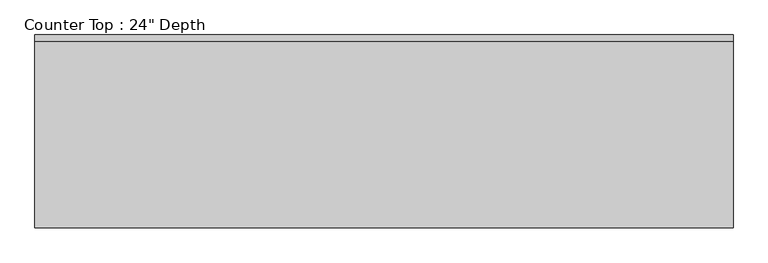
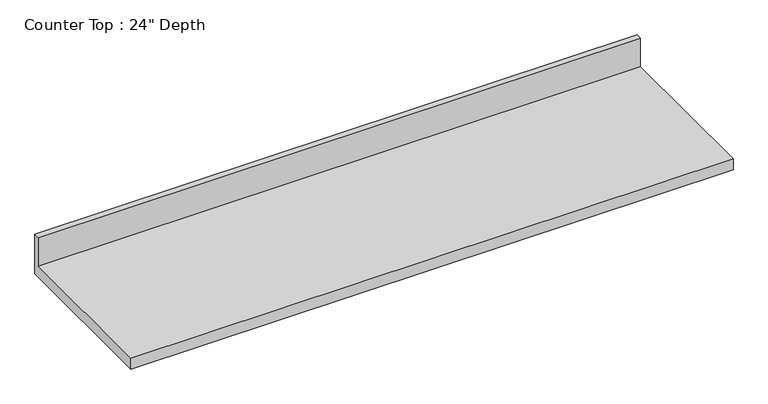
"""IFC4 building model written with IfcOpenShell, lengths in millimetres: furniture geometry."""

from ifc_helpers import new_model, si_unit, frame, origin, place, context, project, spatial, polyline, outline, extrude, source, transform, mapped, element, save


def furniture_a1c4a40b(model_context):
    return source(origin(), model_context, "Body", "SweptSolid", [
        extrude(outline(polyline([(0.0, 1016.0), (0.0, 876.3), (-558.8, 876.3), (-558.8, 914.4), (-19.05, 914.4), (-19.05, 1016.0), (0.0, 1016.0)])), frame((-1200.4622951, 0.0, 0.0), z_axis=(1.0, 0.0, 0.0), x_axis=(0.0, 1.0, 0.0)), (0.0, 0.0, 1.0), 2024.0625),
    ])


if __name__ == "__main__":
    model = new_model("IFC4")
    model_context = context("Model", 3, world=origin())
    ifc_project = project(units=[si_unit("LENGTHUNIT", "METRE", prefix="MILLI")], contexts=[model_context])
    site = spatial("IfcSite", under=ifc_project)
    building = spatial("IfcBuilding", under=site)
    placement = place(None, origin())
    furniture_shape = furniture_a1c4a40b(model_context)
    element("IfcFurniture", 1, ObjectType="Counter Top : 24\" Depth", at=placement, inside=building, context=model_context, shape_type="MappedRepresentation", body=[
        mapped(furniture_shape, transform((0.0, 0.0, 0.0), x_axis=(1.0, 0.0, 0.0), y_axis=(0.0, 1.0, 0.0), z_axis=(0.0, 0.0, 1.0))),
    ])
    save(model, "model.ifc")

# Revit data of these elements
# Type "Counter Top : 24\" Depth"
#   Keynote = "M12366116.01"
#   Assembly Code = "C1030400"
#   Counter Thickness = 0' - 1 1/2"
#   Depth = 1' - 10"
#   Height = 3' - 0"
#   Length [instance default] = 8' - 0"
#   Counter Top Material = none
# Element 1 (IfcFurniture, "Counter Top : 24\" Depth")
#   Length = 6' - 7 11/16"
